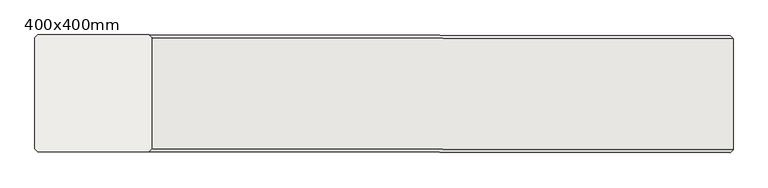
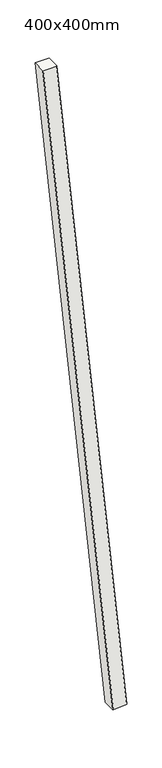
"""IFC4 building model written with IfcOpenShell, lengths in millimetres: slab geometry, CO_01_001_Geheide_prefab_betonpaal : 400x400mm."""

from ifc_helpers import new_model, si_unit, origin, place, context, project, spatial, faceted_brep, source, transform, mapped, element, save


def slab_400x400mm_176eb299(model_context):
    return source(origin(), model_context, "Body", "Brep", [
        faceted_brep([(2179.0570661, -200.0, -22481.0942934), (1800.9429339, -200.0, -22518.9057066), (1790.992562, -190.0, -22519.9007438), (1790.992562, 190.0, -22519.9007438), (1800.9429339, 200.0, -22518.9057066), (2179.0570661, 200.0, -22481.0942934), (2189.007438, 190.0, -22480.0992562), (2189.007438, -190.0, -22480.0992562), (200.9975124, -190.0, -2600.0), (190.9476368, -200.0, -2600.0), (200.9975124, 190.0, -2600.0), (190.9476368, 200.0, -2600.0), (-190.9476368, 200.0, -2600.0), (-200.9975124, 190.0, -2600.0), (-200.9975124, -190.0, -2600.0), (-190.9476368, -200.0, -2600.0)], [[[0, 1, 2, 3, 4, 5, 6, 7]], [[0, 7, 8, 9]], [[7, 6, 10, 8]], [[6, 5, 11, 10]], [[5, 4, 12, 11]], [[4, 3, 13, 12]], [[3, 2, 14, 13]], [[2, 1, 15, 14]], [[1, 0, 9, 15]], [[9, 8, 10, 11, 12, 13, 14, 15]]]),
    ])


if __name__ == "__main__":
    model = new_model("IFC4")
    model_context = context("Model", 3, world=origin())
    ifc_project = project(units=[si_unit("LENGTHUNIT", "METRE", prefix="MILLI")], contexts=[model_context])
    site = spatial("IfcSite", under=ifc_project)
    building = spatial("IfcBuilding", under=site)
    placement = place(None, origin())
    slab_400x400mm_shape = slab_400x400mm_176eb299(model_context)
    element("IfcSlab", 1, ObjectType="CO_01_001_Geheide_prefab_betonpaal : 400x400mm", at=placement, inside=building, context=model_context, shape_type="MappedRepresentation", body=[
        mapped(slab_400x400mm_shape, transform((0.0, 0.0, 0.0), x_axis=(1.0, 0.0, 0.0), y_axis=(0.0, 1.0, 0.0), z_axis=(0.0, 0.0, 1.0))),
    ])
    save(model, "model.ifc")

# Revit data of these elements
# Project information
#   Organization Name = "Dura Vermeer"
#   Organization Description = "Revit Template"
#   Building Name = "2022.3"
#   Author = "JVL"
#   Project Status = "Voorlopig Ontwerp"
#   Client Name = "OPDRACHTGEVER"
#   Project Address = "Taurusavenue 100\n2132LS Hoofddorp"
#   Project Name = "Test Template DVI"
# Type "CO_01_001_Geheide_prefab_betonpaal : 400x400mm"
#   Carbon_Emission_Factor_kgCO2e_per_m = "95"
#   Omschrijving = "Geheide prefab betonpaal; 400x400mm"
#   Description = "Driven precast concrete pile; 400x400mm"
#   CHECK_paallengte [instance default] = "geen problemen"
#   CHECK_raker [instance default] = "geen problemen"
#   Assembly Code = "CO_01_001"
#   Schoorstand_.._1 [instance default] = 5
#   Max_lengte = 36000 mm
#   CALC_WidthNeg [instance default] = -400 mm
#   Width = 400 mm
#   CALC_Vert Pile Length [instance default] = 2250 mm
#   Vellingkant = 10 mm
#   CALC_Top Level [instance default] = 150 mm
#   CALC_asInput_ToeLevel [instance default] = 2250 mm
#   Schoorstand_graden [instance default] = 78.6901°
#   Schoorstand_1_ [instance default] = 0.2
#   Onderkant [instance default] = -1500 mm
#   Lengte [instance default] = 2549.51 mm
#   Bovenkant_tov_NAP [instance default] = 1000 mm
#   Onderkant_tov_NAP [instance default] = -1500 mm
#   CALC_Slopedist cut off [instance default] = 50.99 mm
#   CALC_Slopedist bottom [instance default] = 450 mm
#   CALC_Slopedist Toe Level [instance default] = 450 mm
#   CALC_Slopedist Pile length [instance default] = 450 mm
#   CALC_Refplane Top [instance default] = 900 mm
#   CALC_Rakersymbol rotation [instance default] = 90.00°
#   Schoorsymbool_rotatie [instance default] = 0.00°
#   CALC_Rakersymbol Offset [instance default] = 200 mm
#   CALC_asInput_PileLength [instance default] = -254.951 mm
#   Lengte_paal [instance default] = 0 mm
#   CALC_FlatcutExtention_height [instance default] = 100 mm
#   CALC_FlatcutExtention_dist [instance default] = 20 mm
#   CALC_CutOff [instance default] = 254.951 mm
#   Bovenkant [instance default] = 1000 mm
#   Afhak_hoogte_tov_NAP [instance default] = 750 mm
#   Rakertext Rotate 90deg [instance default] = no
#   Rakertext Rotate 270deg [instance default] = no
#   Rakertext Rotate 180deg [instance default] = no
#   Rakertext Rotate 0deg [instance default] = yes
#   RakerSymbol_vis [instance default] = yes
#   Paal_per_lengte [instance default] = no
#   Cut off_vis [instance default] = yes
#   Pile Symbol = element 2909614
#   Structural Material = none
#   Length = 0
# Element 1 (IfcSlab, "CO_01_001_Geheide_prefab_betonpaal : 400x400mm")
#   Schoorstand_.._1 = 10
#   CALC_Vert Pile Length = 19900 mm
#   CALC_Top Level = 2750 mm
#   CALC_asInput_ToeLevel = 19900 mm
#   Schoorstand_graden = 84.2894°
#   Schoorstand_1_ = 0.1
#   Onderkant = -22500 mm
#   Lengte = 19999.252 mm
#   Bovenkant_tov_NAP = -2600 mm
#   Onderkant_tov_NAP = -22500 mm
#   CALC_Slopedist cut off = 0 mm
#   CALC_Slopedist bottom = 1990 mm
#   CALC_Slopedist Toe Level = 1990 mm
#   CALC_Slopedist Pile length = 1990 mm
#   CALC_Refplane Top = 150 mm
#   CALC_asInput_PileLength = 0 mm
#   CALC_FlatcutExtention_dist = 10 mm
#   CALC_CutOff = 0 mm
#   Bovenkant = -2600 mm
#   Afhak_hoogte_tov_NAP = -2600 mm
#   Cut off_vis = no
#   Materials on its faces: "Beton_Prefab"
# Materials
#   "Beton_Prefab": class "Beton", colour RGB 192 192 192, transparency 0, Description = "NL_Infra", Cost = 0
